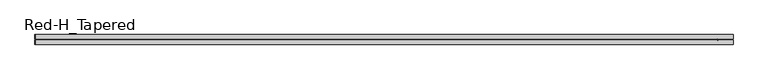
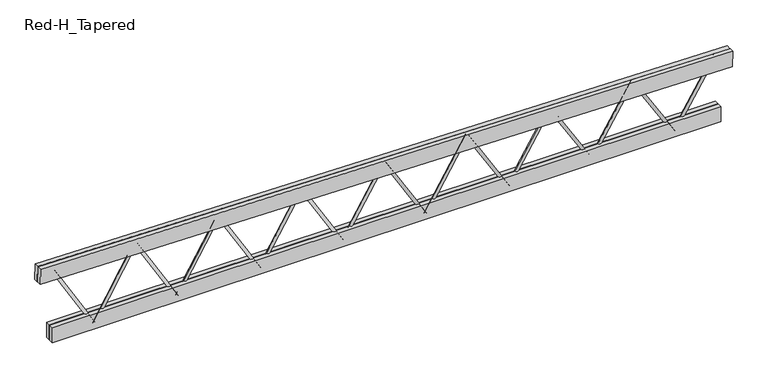
"""IFC4 building model written with IfcOpenShell, lengths in millimetres: beam geometry, Construction_Frames_RedBuilt_Openweb_Red-H_Tapered : Red-H_Tapered."""

from ifc_helpers import new_model, si_unit, point, frame, origin, origin_2d, place, context, project, spatial, polyline, circle_curve, trimmed, segment, composite_curve, outline, extrude, source, transform, mapped, element, save


def red_h_tapered_3106319d(model_context):
    return source(origin(), model_context, "Body", "SweptSolid", [
        extrude(outline(composite_curve([segment(trimmed(circle_curve(origin_2d(), 12.7), [point((0.0, 12.7))], [point((0.0, -12.7))], False, "CARTESIAN"), True, "CONTINUOUS"), segment(trimmed(circle_curve(origin_2d(), 12.7), [point((0.0, -12.7))], [point((0.0, 12.7))], False, "CARTESIAN"), True, "CONTINUOUS")], self_intersect=False)), frame((2514.6356775, 0.0, -367.0101562), z_axis=(0.5238075847033234, 0.0, 0.8518366123895301), x_axis=(0.0, -1.0, 0.0)), (0.0, 0.0, 1.0), 685.812269),
        extrude(outline(composite_curve([segment(trimmed(circle_curve(origin_2d(), 12.7), [point((0.0, -12.7))], [point((0.0, 12.6999999))], False, "CARTESIAN"), True, "CONTINUOUS"), segment(trimmed(circle_curve(origin_2d(), 12.7), [point((0.0, 12.6999999))], [point((0.0, -12.7))], False, "CARTESIAN"), True, "CONTINUOUS")], self_intersect=False)), frame((2514.6356775, 0.0, -367.0101562), z_axis=(-0.5212365661564216, 0.0, 0.8534122345627947), x_axis=(0.0, -1.0, 0.0)), (0.0, 0.0, 1.0), 689.1950633),
        extrude(outline(composite_curve([segment(trimmed(circle_curve(origin_2d(), 12.7), [point((0.0, 12.7))], [point((0.0, -12.6999999))], False, "CARTESIAN"), True, "CONTINUOUS"), segment(trimmed(circle_curve(origin_2d(), 12.7), [point((0.0, -12.6999999))], [point((0.0, 12.7))], False, "CARTESIAN"), True, "CONTINUOUS")], self_intersect=False)), frame((1796.168341, 0.0, -367.0101562), z_axis=(0.5212365661564208, 0.0, 0.8534122345627951), x_axis=(0.0, -1.0, 0.0)), (0.0, 0.0, 1.0), 689.1950633),
        extrude(outline(composite_curve([segment(trimmed(circle_curve(origin_2d(), 12.7), [point((0.0, -12.7))], [point((0.0, 12.7000001))], False, "CARTESIAN"), True, "CONTINUOUS"), segment(trimmed(circle_curve(origin_2d(), 12.7), [point((0.0, 12.7000001))], [point((0.0, -12.7))], False, "CARTESIAN"), True, "CONTINUOUS")], self_intersect=False)), frame((1796.168341, 0.0, -367.0101562), z_axis=(-0.5186860157662654, 0.0, 0.854964804567134), x_axis=(0.0, -1.0, 0.0)), (0.0, 0.0, 1.0), 692.584063),
        extrude(outline(composite_curve([segment(trimmed(circle_curve(origin_2d(), 12.7), [point((0.0, 12.7))], [point((0.0, -12.7))], False, "CARTESIAN"), True, "CONTINUOUS"), segment(trimmed(circle_curve(origin_2d(), 12.7), [point((0.0, -12.7))], [point((0.0, 12.7))], False, "CARTESIAN"), True, "CONTINUOUS")], self_intersect=False)), frame((1077.7010046, 0.0, -367.0101562), z_axis=(0.5186860157662644, 0.0, 0.8549648045671345), x_axis=(0.0, -1.0, 0.0)), (0.0, 0.0, 1.0), 692.584063),
        extrude(outline(composite_curve([segment(trimmed(circle_curve(origin_2d(), 12.7), [point((0.0, -12.7))], [point((0.0, 12.7))], False, "CARTESIAN"), True, "CONTINUOUS"), segment(trimmed(circle_curve(origin_2d(), 12.7), [point((0.0, 12.7))], [point((0.0, -12.7))], False, "CARTESIAN"), True, "CONTINUOUS")], self_intersect=False)), frame((1077.7010046, 0.0, -367.0101562), z_axis=(-0.5161557699811348, 0.0, 0.8564947291812028), x_axis=(0.0, -1.0, 0.0)), (0.0, 0.0, 1.0), 695.9791774),
        extrude(outline(composite_curve([segment(trimmed(circle_curve(origin_2d(), 12.7), [point((0.0, 12.7))], [point((0.0, -12.7))], False, "CARTESIAN"), True, "CONTINUOUS"), segment(trimmed(circle_curve(origin_2d(), 12.7), [point((0.0, -12.7))], [point((0.0, 12.7))], False, "CARTESIAN"), True, "CONTINUOUS")], self_intersect=False)), frame((359.2336682, 0.0, -367.0101562), z_axis=(0.5161557699811353, 0.0, 0.8564947291812025), x_axis=(0.0, -1.0, 0.0)), (0.0, 0.0, 1.0), 695.9791774),
        extrude(outline(composite_curve([segment(trimmed(circle_curve(origin_2d(), 12.7), [point((0.0, -12.7000001))], [point((0.0, 12.7))], False, "CARTESIAN"), True, "CONTINUOUS"), segment(trimmed(circle_curve(origin_2d(), 12.7), [point((0.0, 12.7))], [point((0.0, -12.7000001))], False, "CARTESIAN"), True, "CONTINUOUS")], self_intersect=False)), frame((359.2336682, 0.0, -367.0101562), z_axis=(-0.5136456648662082, 0.0, 0.8580024073183892), x_axis=(0.0, -1.0, 0.0)), (0.0, 0.0, 1.0), 699.3803176),
        extrude(outline(composite_curve([segment(trimmed(circle_curve(origin_2d(), 12.7), [point((0.0, -12.7))], [point((0.0, 12.7000001))], False, "CARTESIAN"), True, "CONTINUOUS"), segment(trimmed(circle_curve(origin_2d(), 12.7), [point((0.0, 12.7000001))], [point((0.0, -12.7))], False, "CARTESIAN"), True, "CONTINUOUS")], self_intersect=False)), frame((-359.2336682, 0.0, -367.0101562), z_axis=(0.5136456648661768, 0.0, 0.858002407318408), x_axis=(0.0, -1.0, 0.0)), (0.0, 0.0, 1.0), 699.3803176),
        extrude(outline(composite_curve([segment(trimmed(circle_curve(origin_2d(), 12.7), [point((0.0, 12.7))], [point((0.0, -12.7))], False, "CARTESIAN"), True, "CONTINUOUS"), segment(trimmed(circle_curve(origin_2d(), 12.7), [point((0.0, -12.7))], [point((0.0, 12.7))], False, "CARTESIAN"), True, "CONTINUOUS")], self_intersect=False)), frame((-359.2336682, 0.0, -367.0101562), z_axis=(-0.5111555362037679, 0.0, 0.8594882301743513), x_axis=(0.0, -1.0, 0.0)), (0.0, 0.0, 1.0), 702.7873959),
        extrude(outline(composite_curve([segment(trimmed(circle_curve(origin_2d(), 12.7), [point((0.0, -12.7000001))], [point((0.0, 12.7))], False, "CARTESIAN"), True, "CONTINUOUS"), segment(trimmed(circle_curve(origin_2d(), 12.7), [point((0.0, 12.7))], [point((0.0, -12.7000001))], False, "CARTESIAN"), True, "CONTINUOUS")], self_intersect=False)), frame((-1077.7010046, 0.0, -367.0101562), z_axis=(0.5111555362037662, 0.0, 0.8594882301743523), x_axis=(0.0, -1.0, 0.0)), (0.0, 0.0, 1.0), 702.7873959),
        extrude(outline(composite_curve([segment(trimmed(circle_curve(origin_2d(), 12.7), [point((0.0, 12.7))], [point((0.0, -12.7))], False, "CARTESIAN"), True, "CONTINUOUS"), segment(trimmed(circle_curve(origin_2d(), 12.7), [point((0.0, -12.7))], [point((0.0, 12.7))], False, "CARTESIAN"), True, "CONTINUOUS")], self_intersect=False)), frame((-1077.7010046, 0.0, -367.0101562), z_axis=(-0.5086852195886402, 0.0, 0.8609525813725497), x_axis=(0.0, -1.0, 0.0)), (0.0, 0.0, 1.0), 706.2003266),
        extrude(outline(composite_curve([segment(trimmed(circle_curve(origin_2d(), 12.7), [point((0.0, -12.7))], [point((0.0, 12.6999999))], False, "CARTESIAN"), True, "CONTINUOUS"), segment(trimmed(circle_curve(origin_2d(), 12.7), [point((0.0, 12.6999999))], [point((0.0, -12.7))], False, "CARTESIAN"), True, "CONTINUOUS")], self_intersect=False)), frame((-1796.168341, 0.0, -367.0101562), z_axis=(0.5086852195886533, 0.0, 0.860952581372542), x_axis=(0.0, -1.0, 0.0)), (0.0, 0.0, 1.0), 706.2003266),
        extrude(outline(composite_curve([segment(trimmed(circle_curve(origin_2d(), 12.7), [point((0.0, 12.6999999))], [point((0.0, -12.7000001))], False, "CARTESIAN"), True, "CONTINUOUS"), segment(trimmed(circle_curve(origin_2d(), 12.7), [point((0.0, -12.7000001))], [point((0.0, 12.6999999))], False, "CARTESIAN"), True, "CONTINUOUS")], self_intersect=False)), frame((-1796.168341, 0.0, -367.0101562), z_axis=(-0.5062345505185007, 0.0, 0.8623958371080716), x_axis=(0.0, -1.0, 0.0)), (0.0, 0.0, 1.0), 709.6190251),
        extrude(outline(composite_curve([segment(trimmed(circle_curve(origin_2d(), 12.7), [point((0.0, -12.6999999))], [point((0.0, 12.7000001))], False, "CARTESIAN"), True, "CONTINUOUS"), segment(trimmed(circle_curve(origin_2d(), 12.7), [point((0.0, 12.7000001))], [point((0.0, -12.6999999))], False, "CARTESIAN"), True, "CONTINUOUS")], self_intersect=False)), frame((-2514.6356775, 0.0, -367.0101562), z_axis=(0.506234550518489, 0.0, 0.8623958371080784), x_axis=(0.0, -1.0, 0.0)), (0.0, 0.0, 1.0), 709.6190251),
        extrude(outline(composite_curve([segment(trimmed(circle_curve(origin_2d(), 12.7), [point((0.0, 12.7))], [point((0.0, -12.7))], False, "CARTESIAN"), True, "CONTINUOUS"), segment(trimmed(circle_curve(origin_2d(), 12.7), [point((0.0, -12.7))], [point((0.0, 12.7))], False, "CARTESIAN"), True, "CONTINUOUS")], self_intersect=False)), frame((-2514.6356775, 0.0, -367.0101562), z_axis=(-0.5038033644797567, 0.0, 0.8638183662893939), x_axis=(0.0, -1.0, 0.0)), (0.0, 0.0, 1.0), 713.0434085),
        extrude(outline(polyline([(-2899.2693457, -41.275), (-2899.2693457, -3.175), (2899.2693457, -3.175), (2899.2693457, -41.275), (-2899.2693457, -41.275)])), frame((0.0, 0.0, -386.0601562), z_axis=(0.0, 0.0, 1.0), x_axis=(1.0, 0.0, 0.0)), (0.0, 0.0, 1.0), 139.7),
        extrude(outline(polyline([(-2899.2693457, 3.175), (-2899.2693457, 41.275), (2899.2693457, 41.275), (2899.2693457, 3.175), (-2899.2693457, 3.175)])), frame((0.0, 0.0, -386.0601562), z_axis=(0.0, 0.0, 1.0), x_axis=(1.0, 0.0, 0.0)), (0.0, 0.0, 1.0), 139.7),
        extrude(outline(polyline([(0.0, -38.1), (0.0, 0.0), (6002.5985939, 0.0), (6002.5985939, -38.1), (0.0, -38.1)])), frame((-3003.2339083, -3.175, 185.4598565), z_axis=(0.016926002698829053, 0.0, 0.9998567449553157), x_axis=(0.9998567449553157, 0.0, -0.016926002698829053)), (0.0, 0.0, 1.0), 139.7),
        extrude(outline(polyline([(0.0, -38.1), (0.0, 0.0), (6002.5985939, 0.0), (6002.5985939, -38.1), (0.0, -38.1)])), frame((-3003.2339083, 41.275, 185.4598565), z_axis=(0.016926002698829053, 0.0, 0.9998567449553157), x_axis=(0.9998567449553157, 0.0, -0.016926002698829053)), (0.0, 0.0, 1.0), 139.7),
    ])


if __name__ == "__main__":
    model = new_model("IFC4")
    model_context = context("Model", 3, world=origin())
    ifc_project = project(units=[si_unit("LENGTHUNIT", "METRE", prefix="MILLI")], contexts=[model_context])
    site = spatial("IfcSite", under=ifc_project)
    building = spatial("IfcBuilding", under=site)
    placement = place(None, origin())
    red_h_tapered_shape = red_h_tapered_3106319d(model_context)
    element("IfcBeam", 1, ObjectType="Construction_Frames_RedBuilt_Openweb_Red-H_Tapered : Red-H_Tapered", at=placement, inside=building, context=model_context, shape_type="MappedRepresentation", body=[
        mapped(red_h_tapered_shape, transform((0.0, 0.0, 0.0), x_axis=(1.0, 0.0, 0.0), y_axis=(0.0, 1.0, 0.0), z_axis=(0.0, 0.0, 1.0))),
    ])
    save(model, "model.ifc")

# Revit data of these elements
# Type "Construction_Frames_RedBuilt_Openweb_Red-H_Tapered : Red-H_Tapered"
#   Youtube clip = ""
#   Weight Net (Kg) = "0"
#   Webs = "Up to 2\" diameter tubular steel"
#   Uniformat II Description = ""
#   Uniformat II Code = ""
#   Uniclass 2015 Name = "Softwood trusses"
#   Uniclass 2015 Code = "Pr_20_85_90_81"
#   Uniclass 2.0 Description = "Structural Framing Systems"
#   Uniclass 2.0 Code = "SS-15-10-75"
#   Uniclass 1.4 Description = "Trusses"
#   Uniclass 1.4 Code = "L3523"
#   UNSPSC Code = "30103606"
#   Technical description = "http://www.redbuilt.com/reference/literature-and-other-resources"
#   Region South America = "None"
#   Region Oceania = "None"
#   Region North America = "US"
#   Region Middle East = "None"
#   Region Europe = "None"
#   Region Asia = "None"
#   Region Antarctica = "None"
#   Region Africa = "None"
#   QR code = "http://bimobject.com/redbuilt/product/redbuilt-0003"
#   Product url = "http://www.redbuilt.com/products/default.aspx?id=2"
#   Product group = "Wood Trusses"
#   Product family = "Construction"
#   Product data url = "https://bimobject.com/redbuilt/product/redbuilt-0003"
#   Product certification = ""
#   Product SKU = "redbuilt-0003"
#   Product Page URL = "http://www.redbuilt.com/commercial-systems/red-m-red-h-open-web-trusses"
#   Product Guid = "2c5793f2-6ffb-4665-b825-cf90c048e711"
#   Product Documentation Link = "http://www.redbuilt.com/documents/OW_Guide_2017_07_LowRes_wLinks.pdf"
#   OmniClass Description = "Wood Trusses"
#   OmniClass Code = "23-13 35 19 13 17"
#   NBS Reference Description = ""
#   NBS Reference Code = ""
#   Material secondary = "Steel"
#   Material main = "CHARRED WOOD"
#   Masterformat 2014 Description = "Metal-Web Wood Joists"
#   Masterformat 2014 Code = "06 17 36"
#   Manufacturer name = "RedBuilt"
#   Manufacturer country = "United States"
#   Installation instructions = "http://www.redbuilt.com/documents/Installation_Sheets_Open-Web.pdf"
#   IFC Classification = ""
#   EAN code = ""
#   Design country = "United States"
#   Product Information = "http://redbuilt.com/products/default.aspx?id=2"
#   Model = "Red-H-Tapered"
#   Manufacturer URL = "http://redbuilt.com/"
#   Manufacturer = "RedBuilt™"
#   Description = "Open Web Truss"
#   Date of publishing = "8/17/2010"
#   Contact us = "http://redbuilt.com/contact/"
#   Chords = "Double 1½\" x 5½\" MSR lumber"
#   COBIe Type Category = ""
#   Brand url = "http://www.redbuilt.com"
#   BIMobject main category code = "construction"
#   BIMobject main category = "Construction"
#   BIMobject category code = "construction-frames-trusses"
#   BIMobject category = "Frames & Trusses"
#   Web Radius = 0' - 0 1/2"
#   Web Layout Offset Start [instance default] = 0' - 5"
#   Web Layout Offset End [instance default] = 0' - 5"
#   Web Diameter = 0' - 1"
#   TotalLength [instance default] = 20' - 0"
#   Span Minimum = 4' - 0"
#   Span Maximum = 70' - 0"
#   Span Limit [instance default] = 20' - 0"
#   Nominal width = 0' - 0"
#   Nominal height = 0' - 0"
#   Inner Depth Top [instance default] = 0' - 2.76372"
#   Depth Start [instance default] = 6' - 0"
#   Top Chord Length [instance default] = 20' - 1.19701"
#   TC Extension Start Aux [instance default] = 0' - 0"
#   TC Extension End Aux [instance default] = 0' - 0"
#   T-B Chord Length Difference L [instance default] = 0' - 4"
#   T-B Chord Length Difference [instance default] = 0' - 4"
#   Height 2 [instance default] = 6' - 0"
#   Depth Minimum at Wall = 2' - 0"
#   Depth Maximum at Wall = 6' - 0"
#   Depth Lower End [instance default] = 2' - 0"
#   Depth Higher End [instance default] = 6' - 0"
#   Depth End [instance default] = 2' - 0"
#   Depth 2 [instance default] = 2' - 0"
#   Chord Width = 0' - 3 1/4"
#   Chord Thickness = 0' - 1 1/2"
#   Chord Depth = 0' - 5 1/2"
#   Offset Start [instance default] = 0' - 0"
#   TC Extension Start [instance default] = 0' - 0"
#   End Panel = 0' - 5"
#   Offset End [instance default] = 0' - 0"
#   TC Extension End [instance default] = 0' - 0"
#   Length [instance default] = 20' - 0"
#   Angle [instance default] = 5.71059°
#   Span Limit Warning [instance default] = no
#   Edition number = 1
#   Top Bearing Start [instance default] = yes
#   Top Bearing End [instance default] = yes
#   Bottom Bearing Start [instance default] = no
#   Bottom Bearing End [instance default] = no
#   8 Panels [instance default] = yes
#   16 Panels [instance default] = no
#   12 Panels [instance default] = no
#   Web Material = RedBuilt-Steel, Galvanized
#   Clip Material = RedBuilt-Steel, Galvanized
#   Chords Material = WOOD-OAKFIRE
#   URL = ""
#   Assembly Code = ""
# Element 1 (IfcBeam, "Construction_Frames_RedBuilt_Openweb_Red-H_Tapered : Red-H_Tapered")
#   TotalLength = 19' - 8.28892"
#   Span Limit = 19' - 8.28892"
#   Inner Depth Top = 0' - 2.75039"
#   Depth Start = 5' - 0"
#   Top Chord Length = 19' - 8.32278"
#   Height 2 = 5' - 0"
#   Depth Higher End = 5' - 0"
#   Depth 2 = 0' - 4"
#   Angle = 0.969835°
#   Materials on its faces: "RedBuilt-Steel, Galvanized", "WOOD-OAKFIRE"
# Materials
#   "RedBuilt-Steel, Galvanized": class "Metal", colour RGB 164 172 176, transparency 0, Manufacturer = "RedBuilt. LLC", Comments = "Openweb Metal Web", URL = "http://www.redbuilt.com/", Description = "Galvanized steel", Cost = 0
#   "WOOD-OAKFIRE": class "Wood", colour RGB 198 202 183, transparency 0, Description = "Generic wood", Cost = 0
